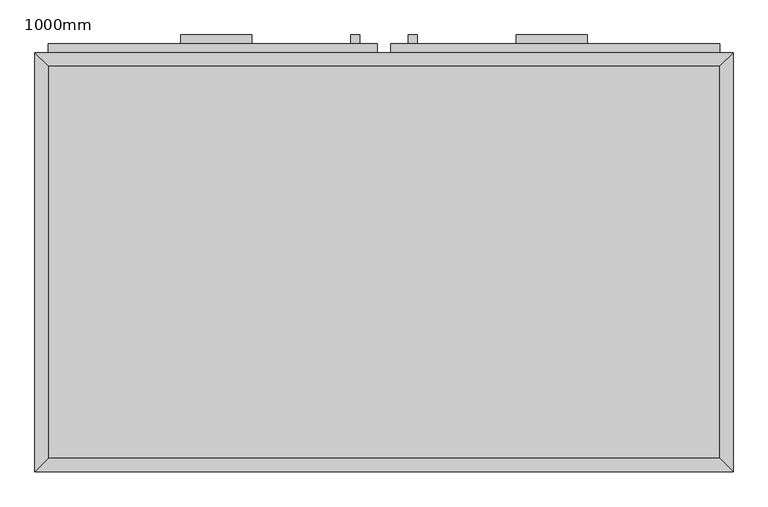
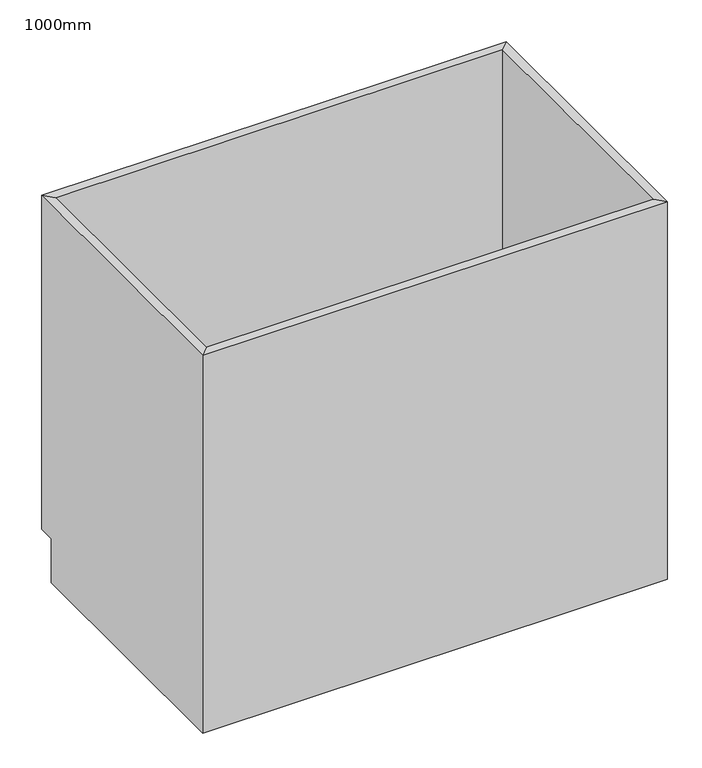
"""IFC4 building model written with IfcOpenShell, lengths in millimetres: furniture geometry, M_Base Cabinet-Double Door & 2 Drawer : 1000mm."""

import ifcopenshell
import ifcopenshell.guid

model = None  # the IFC model being written
_history = None  # IfcOwnerHistory: only IFC2X3 demands one
_inside = {}  # id of a spatial element -> (the spatial element, [elements in it])
_under = {}  # id of a project, library or spatial element -> (it, [spatial elements below it])
_declared = {}  # id of a project -> (the project, [libraries it declares])
_typed = {}  # id of a type object -> (the type object, [elements of that type])
_made_of = {}  # id of a material, layer set ... -> (it, [elements and type objects made of it])


def new_model(schema):
    """Start an empty IFC model of exactly this schema.

    Asked for "IFC4X3", IfcOpenShell would pick the latest addendum, in which some entities
    have other attributes; the version numbers below select the first issue.
    IFC2X3 requires an IfcOwnerHistory on every rooted entity: one is made here for all.
    """
    global model, _history
    if schema == "IFC4X3":
        model = ifcopenshell.file(schema_version=(4, 3, 0, 0))
    else:
        model = ifcopenshell.file(schema=schema)
    _inside.clear()
    _under.clear()
    _declared.clear()
    _typed.clear()
    _made_of.clear()
    _history = None
    if model.schema == "IFC2X3":
        org = make("IfcOrganization", Name="unknown")
        user = make(
            "IfcPersonAndOrganization",
            ThePerson=make("IfcPerson", FamilyName="unknown"),
            TheOrganization=org,
        )
        app = make(
            "IfcApplication",
            ApplicationDeveloper=org,
            Version="unknown",
            ApplicationFullName="unknown",
            ApplicationIdentifier="unknown",
        )
        _history = make(
            "IfcOwnerHistory",
            OwningUser=user,
            OwningApplication=app,
            ChangeAction="ADDED",
            CreationDate=0,
        )
    return model


def make(cls, **values):
    """One entity of the class cls with the attributes given. An attribute that is None is left unset."""
    return model.create_entity(
        cls, **{name: value for name, value in values.items() if value is not None}
    )


def rooted(cls, **values):
    """An entity with a GlobalId (a new one), such as an element, a storey or a relation."""
    return make(cls, GlobalId=ifcopenshell.guid.new(), OwnerHistory=_history, **values)


def si_unit(unit_type, name, prefix=None):
    """IfcSIUnit, for example si_unit("LENGTHUNIT", "METRE", prefix="MILLI")."""
    return make("IfcSIUnit", UnitType=unit_type, Prefix=prefix, Name=name)


def assignment(units):
    """IfcUnitAssignment: the units of a project."""
    return None if units is None else make("IfcUnitAssignment", Units=units)


def point(xyz):
    """IfcCartesianPoint."""
    return None if xyz is None else make("IfcCartesianPoint", Coordinates=xyz)


def direction(xyz):
    """IfcDirection."""
    return None if xyz is None else make("IfcDirection", DirectionRatios=xyz)


def frame(location, z_axis=None, x_axis=None):
    """IfcAxis2Placement3D, a coordinate frame: its origin and axes. An axis left out is left unset."""
    return make(
        "IfcAxis2Placement3D",
        Location=point(location),
        Axis=direction(z_axis),
        RefDirection=direction(x_axis),
    )


def origin():
    """The frame at (0, 0, 0) with its axes left unset."""
    return frame((0.0, 0.0, 0.0))


def place(relative_to, where):
    """IfcLocalPlacement: puts the frame where relative to a parent placement (None: the world)."""
    return make(
        "IfcLocalPlacement", PlacementRelTo=relative_to, RelativePlacement=where
    )


def context(
    kind, dimensions, precision=None, world=None, true_north=None, identifier=None
):
    """IfcGeometricRepresentationContext, for example the 3D "Model" context."""
    return make(
        "IfcGeometricRepresentationContext",
        ContextIdentifier=identifier,
        ContextType=kind,
        CoordinateSpaceDimension=dimensions,
        Precision=precision,
        WorldCoordinateSystem=world,
        TrueNorth=true_north,
    )


def project(units=None, contexts=None):
    """IfcProject with its units and contexts."""
    return rooted(
        "IfcProject",
        Name="project",
        RepresentationContexts=contexts,
        UnitsInContext=assignment(units),
    )


def spatial(cls, under=None, at=None, **own):
    """A site, building, storey or space (cls), placed at a placement, below another one or the project."""
    s = rooted(cls, ObjectPlacement=at, **own)
    if under is not None:
        _under.setdefault(under.id(), (under, []))[1].append(s)
    return s


def polyline(points):
    """IfcPolyline through the points."""
    return make("IfcPolyline", Points=[point(p) for p in points])


def outline(outer, holes=None, kind="AREA"):
    """IfcArbitraryClosedProfileDef: a profile drawn as a closed curve; with holes, ...WithVoids."""
    if holes is None:
        return make("IfcArbitraryClosedProfileDef", ProfileType=kind, OuterCurve=outer)
    return make(
        "IfcArbitraryProfileDefWithVoids",
        ProfileType=kind,
        OuterCurve=outer,
        InnerCurves=holes,
    )


def extrude(swept, where, along, depth):
    """IfcExtrudedAreaSolid: the profile swept, set in the frame where, extruded along a direction by depth."""
    return make(
        "IfcExtrudedAreaSolid",
        SweptArea=swept,
        Position=where,
        ExtrudedDirection=direction(along),
        Depth=depth,
    )


def faces_of(points, faces, orient=None, outer=None):
    """IfcFace entities. A face is a list of loops; a loop is a list of indices into points, from 0.

    orient and outer hold one flag for each loop. By default every Orientation is true, the
    first loop of a face is its IfcFaceOuterBound and the others are IfcFaceBound.
    """
    made = []
    for i, loops in enumerate(faces):
        bounds = []
        for j, loop in enumerate(loops):
            is_outer = j == 0 if outer is None else outer[i][j]
            bounds.append(
                make(
                    "IfcFaceOuterBound" if is_outer else "IfcFaceBound",
                    Bound=make("IfcPolyLoop", Polygon=[points[k] for k in loop]),
                    Orientation=True if orient is None else orient[i][j],
                )
            )
        made.append(make("IfcFace", Bounds=bounds))
    return made


def faceted_brep(points, faces, orient=None, outer=None, voids=None):
    """IfcFacetedBrep: a solid bounded by flat faces; with voids (closed shells), ...WithVoids."""
    shared = [point(p) for p in points]
    hull = make("IfcClosedShell", CfsFaces=faces_of(shared, faces, orient, outer))
    if voids is None:
        return make("IfcFacetedBrep", Outer=hull)
    return make(
        "IfcFacetedBrepWithVoids",
        Outer=hull,
        Voids=[
            make(cls, CfsFaces=faces_of(shared, fs, o, b)) for cls, fs, o, b in voids
        ],
    )


def shape(context_of_items, identifier, shape_type, items):
    """IfcShapeRepresentation: the items that make up one representation, for example the "Body"."""
    return make(
        "IfcShapeRepresentation",
        ContextOfItems=context_of_items,
        RepresentationIdentifier=identifier,
        RepresentationType=shape_type,
        Items=items,
    )


def source(mapping_origin, context_of_items, identifier, shape_type, items):
    """IfcRepresentationMap: a shape defined once, which mapped items show again and again."""
    return make(
        "IfcRepresentationMap",
        MappingOrigin=mapping_origin,
        MappedRepresentation=shape(context_of_items, identifier, shape_type, items),
    )


def transform(
    local_origin,
    x_axis=None,
    y_axis=None,
    z_axis=None,
    scale=None,
    scale2=None,
    scale3=None,
    uniform=True,
):
    """IfcCartesianTransformationOperator3D, or its non-uniform kind. x_axis, y_axis, z_axis: its Axis1, 2, 3."""
    if uniform:
        return make(
            "IfcCartesianTransformationOperator3D",
            Axis1=direction(x_axis),
            Axis2=direction(y_axis),
            LocalOrigin=point(local_origin),
            Scale=scale,
            Axis3=direction(z_axis),
        )
    return make(
        "IfcCartesianTransformationOperator3DnonUniform",
        Axis1=direction(x_axis),
        Axis2=direction(y_axis),
        LocalOrigin=point(local_origin),
        Scale=scale,
        Axis3=direction(z_axis),
        Scale2=scale2,
        Scale3=scale3,
    )


def mapped(mapping_source, mapping_target):
    """IfcMappedItem: shows the shape of a source again, moved by a transform."""
    return make(
        "IfcMappedItem", MappingSource=mapping_source, MappingTarget=mapping_target
    )


def made_of(thing, what):
    """Note that an element or type object is made of a material, layer set ...; save() writes the relation."""
    if what is not None:
        _made_of.setdefault(what.id(), (what, []))[1].append(thing)
    return thing


def element(
    cls,
    number,
    at=None,
    inside=None,
    cuts=None,
    type_object=None,
    material=None,
    context=None,
    identifier="Body",
    shape_type=None,
    held_by="IfcProductDefinitionShape",
    body=None,
    shapes=None,
    **own,
):
    """One element of the class cls, such as IfcWall. Its Tag is "e" and its number.

    at: its placement. inside: the storey or other place that contains it. cuts: it is an
    opening in that element (IfcRelVoidsElement). A single representation is given by context,
    identifier, shape_type and body (its items); several are given by shapes. held_by: the class
    of the entity that holds the representations. save() writes the other relations.
    """
    e = rooted(cls, Tag="e%d" % number, ObjectPlacement=at, **own)
    if body is not None:
        shapes = [shape(context, identifier, shape_type, body)]
    if shapes is not None:
        e.Representation = make(held_by, Representations=shapes)
    if inside is not None:
        _inside.setdefault(inside.id(), (inside, []))[1].append(e)
    if cuts is not None:
        rooted(
            "IfcRelVoidsElement", RelatingBuildingElement=cuts, RelatedOpeningElement=e
        )
    if type_object is not None:
        _typed.setdefault(type_object.id(), (type_object, []))[1].append(e)
    return made_of(e, material)


def aggregate(whole, parts):
    """IfcRelAggregates: a whole, such as a stair, and the parts it consists of."""
    return rooted("IfcRelAggregates", RelatingObject=whole, RelatedObjects=parts)


def save(model, path):
    """Write the relations noted so far, then the file.

    IfcRelAggregates (storeys below a building ...), IfcRelContainedInSpatialStructure (elements
    in a storey), IfcRelDefinesByType, IfcRelAssociatesMaterial and IfcRelDeclares: one each for
    every whole, place, type object, material and project.
    """
    for whole, parts in _under.values():
        aggregate(whole, parts)
    for where, things in _inside.values():
        rooted(
            "IfcRelContainedInSpatialStructure",
            RelatedElements=things,
            RelatingStructure=where,
        )
    for kind, things in _typed.values():
        rooted("IfcRelDefinesByType", RelatedObjects=things, RelatingType=kind)
    for what, things in _made_of.values():
        rooted("IfcRelAssociatesMaterial", RelatedObjects=things, RelatingMaterial=what)
    for by, libraries in _declared.values():
        rooted("IfcRelDeclares", RelatingContext=by, RelatedDefinitions=libraries)
    model.write(path)


def furniture_1000mm_55825455(model_context):
    return source(origin(), model_context, "Body", "SolidModel", [
        faceted_brep([(499.6877049, 580.95, 860.0), (-462.2122951, 580.95, 860.0), (-462.2122951, 580.95, 100.0), (499.6877049, 580.95, 100.0), (518.7377049, 600.0, 860.0), (-481.2622951, 600.0, 860.0), (518.7377049, 600.0, 100.0), (-481.2622951, 600.0, 100.0), (-462.2122951, 19.05, 860.0), (-462.2122951, 19.05, 100.0), (-462.2122951, 565.0, 100.0), (-481.2622951, 0.0, 860.0), (-481.2622951, 565.0, 100.0), (-481.2622951, 565.0, 0.0), (-481.2622951, 0.0, 0.0), (499.6877049, 19.05, 860.0), (499.6877049, 19.05, 100.0), (518.7377049, 0.0, 860.0), (518.7377049, 0.0, 0.0), (499.6877049, 565.0, 100.0), (518.7377049, 565.0, 0.0), (518.7377049, 565.0, 100.0)], [[[0, 1, 2, 3]], [[0, 4, 5, 1]], [[4, 6, 7, 5]], [[2, 7, 6, 3]], [[1, 8, 9, 10, 2]], [[5, 11, 8, 1]], [[7, 12, 13, 14, 11, 5]], [[2, 10, 12, 7]], [[8, 15, 16, 9]], [[11, 17, 15, 8]], [[14, 18, 17, 11]], [[3, 19, 16, 15, 0]], [[0, 15, 17, 4]], [[4, 17, 18, 20, 21, 6]], [[6, 21, 19, 3]], [[10, 9, 16, 19]], [[18, 14, 13, 20]], [[13, 12, 10, 19, 21, 20]]]),
        extrude(outline(polyline([(-170.9372951, 625.4), (-170.9372951, 612.7), (-272.5372951, 612.7), (-272.5372951, 625.4), (-170.9372951, 625.4)])), frame((0.0, 0.0, 802.85), z_axis=(0.0, 0.0, 1.0), x_axis=(1.0, 0.0, 0.0)), (0.0, 0.0, 1.0), 12.7),
        extrude(outline(polyline([(310.0127049, 625.4), (310.0127049, 612.7), (208.4127049, 612.7), (208.4127049, 625.4), (310.0127049, 625.4)])), frame((0.0, 0.0, 802.85), z_axis=(0.0, 0.0, 1.0), x_axis=(1.0, 0.0, 0.0)), (0.0, 0.0, 1.0), 12.7),
        extrude(outline(polyline([(-16.1872951, 625.4), (-16.1872951, 612.7), (-28.8872951, 612.7), (-28.8872951, 625.4), (-16.1872951, 625.4)])), frame((0.0, 0.0, 580.6), z_axis=(0.0, 0.0, 1.0), x_axis=(1.0, 0.0, 0.0)), (0.0, 0.0, 1.0), 101.6),
        extrude(outline(polyline([(66.3627049, 625.4), (66.3627049, 612.7), (53.6627049, 612.7), (53.6627049, 625.4), (66.3627049, 625.4)])), frame((0.0, 0.0, 580.6), z_axis=(0.0, 0.0, 1.0), x_axis=(1.0, 0.0, 0.0)), (0.0, 0.0, 1.0), 101.6),
        extrude(outline(polyline([(9.2127049, 612.7), (9.2127049, 600.0), (-462.2122951, 600.0), (-462.2122951, 612.7), (9.2127049, 612.7)])), frame((0.0, 0.0, 739.35), z_axis=(0.0, 0.0, 1.0), x_axis=(1.0, 0.0, 0.0)), (0.0, 0.0, 1.0), 101.6),
        extrude(outline(polyline([(499.6877049, 612.7), (499.6877049, 600.0), (28.2627049, 600.0), (28.2627049, 612.7), (499.6877049, 612.7)])), frame((0.0, 0.0, 739.35), z_axis=(0.0, 0.0, 1.0), x_axis=(1.0, 0.0, 0.0)), (0.0, 0.0, 1.0), 101.6),
        extrude(outline(polyline([(9.2127049, 612.7), (9.2127049, 600.0), (-462.2122951, 600.0), (-462.2122951, 612.7), (9.2127049, 612.7)])), frame((0.0, 0.0, 119.05), z_axis=(0.0, 0.0, 1.0), x_axis=(1.0, 0.0, 0.0)), (0.0, 0.0, 1.0), 601.25),
        extrude(outline(polyline([(499.6877049, 612.7), (499.6877049, 600.0), (28.2627049, 600.0), (28.2627049, 612.7), (499.6877049, 612.7)])), frame((0.0, 0.0, 119.05), z_axis=(0.0, 0.0, 1.0), x_axis=(1.0, 0.0, 0.0)), (0.0, 0.0, 1.0), 601.25),
        extrude(outline(polyline([(499.6877049, 19.05), (-462.2122951, 19.05), (-462.2122951, 580.95), (499.6877049, 580.95), (499.6877049, 19.05)])), frame((0.0, 0.0, 100.0), z_axis=(0.0, 0.0, 1.0), x_axis=(1.0, 0.0, 0.0)), (0.0, 0.0, 1.0), 19.05),
    ])


if __name__ == "__main__":
    model = new_model("IFC4")
    model_context = context("Model", 3, world=origin())
    ifc_project = project(units=[si_unit("LENGTHUNIT", "METRE", prefix="MILLI")], contexts=[model_context])
    site = spatial("IfcSite", under=ifc_project)
    building = spatial("IfcBuilding", under=site)
    placement = place(None, origin())
    furniture_1000mm_shape = furniture_1000mm_55825455(model_context)
    element("IfcFurniture", 1, ObjectType="M_Base Cabinet-Double Door & 2 Drawer : 1000mm", at=placement, inside=building, context=model_context, shape_type="MappedRepresentation", body=[
        mapped(furniture_1000mm_shape, transform((0.0, 0.0, 0.0), x_axis=(1.0, 0.0, 0.0), y_axis=(0.0, 1.0, 0.0), z_axis=(0.0, 0.0, 1.0))),
    ])
    save(model, "model.ifc")

# Revit data of these elements
# Type "M_Base Cabinet-Double Door & 2 Drawer : 1000mm"
#   Manufacturer = "Manufacturer"
#   Finish = "Finish"
#   Construction Type = "Construction Type"
#   AccessibilityPerformance = "AccessibilityPerformance"
#   CodePerformance = "CodePerformance"
#   Area = "Area"
#   Color = "Color"
#   Constituents = "Constituents"
#   Features = "Features"
#   Finish = "Finish"
#   Grade = "Grade"
#   Material = "Material"
#   ModelReference = "ModelReference"
#   NominalHeight = "NominalHeight"
#   NominalLength = "NominalLength"
#   NominalWidth = "NominalWidth"
#   ProductionYear = "ProductionYear"
#   Reference = "Reference"
#   Shape = "Shape"
#   Size = "Size"
#   SustainabilityPerformance = "SustainabilityPerformance"
#   WarrantyDescription = "WarrantyDescription"
#   WarrantyDurationLabor = "WarrantyDurationLabor"
#   WarrantyDurationParts = "WarrantyDurationParts"
#   WarrantyGuarantorLabor = "WarrantyGuarantorLabor"
#   WarrantyGuarantorParts = "WarrantyGuarantorParts"
#   ExpectedLife = "ExpectedLife"
#   ReplacementCost = "ReplacementCost"
#   AssetAccountingType = "FIXED"
#   ModelLabel = "ModelLabel"
#   Depth = 0.600 m
#   Height = 0.860 m
#   Plinth Depth = 0.035 m
#   Plinth Height = 0.100 m
#   Width = 1.000 m
#   Cabinet Material = none
#   Door/Drawer Material = none
#   Handle Material = Cabinets - Handles
# Element 1 (IfcFurniture, "M_Base Cabinet-Double Door & 2 Drawer : 1000mm")
#   Materials on its faces: "Cabinets", "Cabinets - Handles"
# Materials
#   "Cabinets - Handles": class "Metal", colour RGB 57 57 57, transparency 0
#   "Cabinets": class "Miscellaneous", colour RGB 249 249 249, transparency 0
